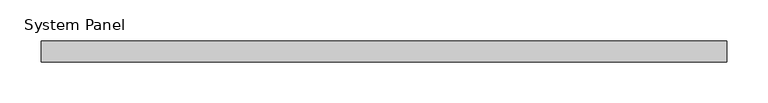
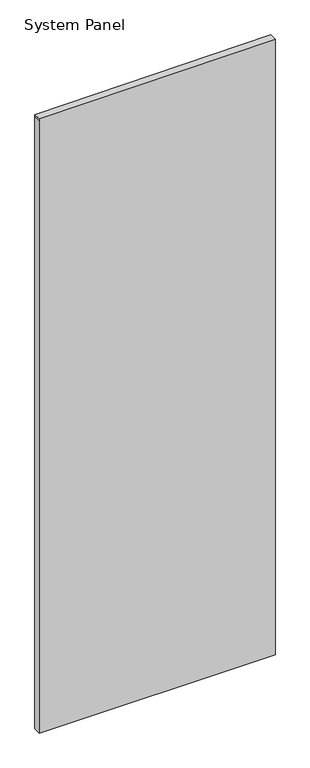
"""IFC4 building model written with IfcOpenShell, lengths in millimetres: plate geometry, System Panel : TEMPERED INSULATED GLAZING (CARDINAL GLASS LoĒ²-240."""

from ifc_helpers import new_model, si_unit, frame, origin, place, context, project, spatial, polyline, outline, extrude, source, transform, mapped, element, save


def system_panel_c44e1770(model_context):
    return source(origin(), model_context, "Body", "SweptSolid", [
        extrude(outline(polyline([(0.0, -416.8619325), (0.0, 416.8619325), (2287.5080968, 416.8619325), (2300.0808528, 416.8619325), (2294.7171056, -416.8619325), (2287.5080968, -416.8619325), (0.0, -416.8619325)])), frame((0.0, -31.75, 0.0), z_axis=(0.0, 1.0, 0.0), x_axis=(0.0, 0.0, 1.0)), (0.0, 0.0, 1.0), 25.4),
    ])


if __name__ == "__main__":
    model = new_model("IFC4")
    model_context = context("Model", 3, world=origin())
    ifc_project = project(units=[si_unit("LENGTHUNIT", "METRE", prefix="MILLI")], contexts=[model_context])
    site = spatial("IfcSite", under=ifc_project)
    building = spatial("IfcBuilding", under=site)
    placement = place(None, origin())
    system_panel_shape = system_panel_c44e1770(model_context)
    element("IfcPlate", 1, ObjectType="System Panel : TEMPERED INSULATED GLAZING (CARDINAL GLASS LoĒ²-240", at=placement, inside=building, context=model_context, shape_type="MappedRepresentation", body=[
        mapped(system_panel_shape, transform((0.0, 0.0, 0.0), x_axis=(1.0, 0.0, 0.0), y_axis=(0.0, 1.0, 0.0), z_axis=(0.0, 0.0, 1.0))),
    ])
    save(model, "model.ifc")

# Revit data of these elements
# Type "System Panel : TEMPERED INSULATED GLAZING (CARDINAL GLASS LoĒ²-240"
#   Construction Type Id = "opn-s72"
#   Analytic Construction = "Double glazing - 1/4 in thick - low-E/clear (e = 0.1) glass"
#   Visual Light Transmittance = 0.72
#   Solar Heat Gain Coefficient = 0.6
#   Heat Transfer Coefficient (U) = 1.9873 W/(m²·K)
#   Transparency_Hack = 70
# Element 1 (IfcPlate, "System Panel : TEMPERED INSULATED GLAZING (CARDINAL GLASS LoĒ²-240")
#   Materials on its faces: "TEMPERED INSULATED GLAZING (CARDINAL GLASS LoĒ²-240\nOR EQUIVALENT)"
# Materials
#   "TEMPERED INSULATED GLAZING (CARDINAL GLASS LoĒ²-240\nOR EQUIVALENT)": class "Glass", colour RGB 196 205 210, transparency 0.85, Description = "Soda Lime Glass", Cost = 0
